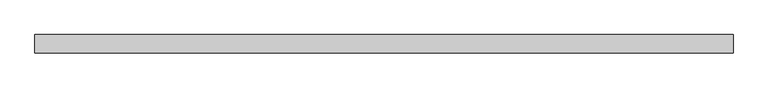
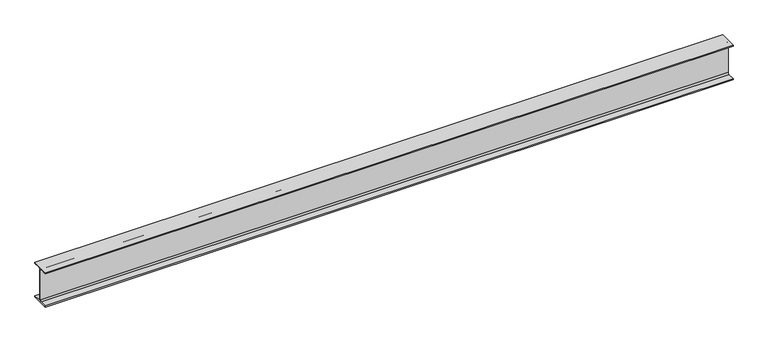
"""IFC4 building model written with IfcOpenShell, lengths in millimetres: beam geometry, 0912_Steel Framing_H-KSD3502 : H_SB_ASB_H-350x175x7x11."""

from ifc_helpers import new_model, si_unit, point, frame, frame_2d, origin, place, context, project, spatial, polyline, circle_curve, trimmed, segment, composite_curve, outline, extrude, source, transform, mapped, element, save


def beam_abbcd3b4(model_context):
    return source(origin(), model_context, "Body", "SweptSolid", [
        extrude(outline(composite_curve([segment(polyline([(87.5, -164.0), (87.5, -175.0), (-87.5, -175.0), (-87.5, -164.0), (-17.5, -164.0)]), True, "CONTINUOUS"), segment(trimmed(circle_curve(frame_2d((-17.5, -150.0)), 14.0), [point((-17.5, -164.0))], [point((-3.5, -150.0))], True, "CARTESIAN"), True, "CONTINUOUS"), segment(polyline([(-3.5, -150.0), (-3.5, 150.0)]), True, "CONTINUOUS"), segment(trimmed(circle_curve(frame_2d((-17.5, 150.0)), 14.0), [point((-3.5, 150.0))], [point((-17.5, 164.0))], True, "CARTESIAN"), True, "CONTINUOUS"), segment(polyline([(-17.5, 164.0), (-87.5, 164.0), (-87.5, 175.0), (87.5, 175.0), (87.5, 164.0), (17.5, 164.0)]), True, "CONTINUOUS"), segment(trimmed(circle_curve(frame_2d((17.5, 150.0)), 14.0), [point((17.5, 164.0))], [point((3.5, 150.0))], True, "CARTESIAN"), True, "CONTINUOUS"), segment(polyline([(3.5, 150.0), (3.5, -150.0)]), True, "CONTINUOUS"), segment(trimmed(circle_curve(frame_2d((17.5, -150.0)), 14.0), [point((3.5, -150.0))], [point((17.5, -164.0))], True, "CARTESIAN"), True, "CONTINUOUS"), segment(polyline([(17.5, -164.0), (87.5, -164.0)]), True, "CONTINUOUS")], self_intersect=False)), frame((-3262.3, 0.0, 0.0), z_axis=(1.0, 0.0, 0.0), x_axis=(0.0, 1.0, 0.0)), (0.0, 0.0, 1.0), 6599.6),
    ])


if __name__ == "__main__":
    model = new_model("IFC4")
    model_context = context("Model", 3, world=origin())
    ifc_project = project(units=[si_unit("LENGTHUNIT", "METRE", prefix="MILLI")], contexts=[model_context])
    site = spatial("IfcSite", under=ifc_project)
    building = spatial("IfcBuilding", under=site)
    placement = place(None, origin())
    beam_shape = beam_abbcd3b4(model_context)
    element("IfcBeam", 1, ObjectType="0912_Steel Framing_H-KSD3502 : H_SB_ASB_H-350x175x7x11", at=placement, inside=building, context=model_context, shape_type="MappedRepresentation", body=[
        mapped(beam_shape, transform((0.0, 0.0, 0.0), x_axis=(1.0, 0.0, 0.0), y_axis=(0.0, 1.0, 0.0), z_axis=(0.0, 0.0, 1.0))),
    ])
    save(model, "model.ifc")

# Revit data of these elements
# Type "0912_Steel Framing_H-KSD3502 : H_SB_ASB_H-350x175x7x11"
#   H_WM Code_1 = "S01AA002-00001 | Main Steel Structure Fabrication Work | Shelter/Building | Medium Steel - Standard (90KG/M>Weight≥30KG/M) | Material: (   )"
#   H_WM Code_2 = "S03AA028-00001 | Main Steel Structure Erection Work | Shelter/Building | Medium Steel (90KG/M>Weight≥30KG/M) | Material: (   )"
#   H_WM Code_3 = "S01AA010-00001 | Main Steel Structure Fabrication Work | Shelter/Building | Steel Painting/Coating | for Non-Fireproofed Steel Surface, Surface Preparation, Primer, Second & Final Coat | Material: (   )"
#   H_Q'ty Cal Type Tag = "SB-Q2"
#   Width = 17.5 cm
#   Web Thickness = 0.7 cm
#   Web Fillet = 1.4 cm
#   Warping Constant = 282000.0 cm⁶
#   W = 0
#   Torsional Moment of Inertia = 19.4042 cm⁴
#   Section Area = 63.14 cm²
#   Plastic Modulus weak axis = 174.0 cm³
#   Plastic Modulus strong axis = 868.0 cm³
#   Perimeter = 1.36 m²/m
#   Nominal Weight = 49.60 kgf/m
#   Moment of Inertia weak axis = 984.00 cm⁴
#   Moment of Inertia strong axis = 13600.00 cm⁴
#   Height = 35.0 cm
#   Flange Thickness = 1.1 cm
#   Elastic Modulus weak axis = 112.0 cm³
#   Elastic Modulus strong axis = 775.0 cm³
#   Centroid Vertical = 17.5 cm
#   Centroid Horizontal = 8.75 cm
#   Ix = 136000000
#   Length [instance default] = 1.5240 m
#   Zx = 868000
#   b = 0.1750 m
#   h = 0.3500 m
#   r = 0.0140 m
#   s = 0.0070 m
#   t = 0.0110 m
#   A = 0.006314 m²
#   Structural Material [instance default] = Steel, 45-345
#   Assembly Code = ""
# Element 1 (IfcBeam, "0912_Steel Framing_H-KSD3502 : H_SB_ASB_H-350x175x7x11")
#   Structural Material = none
# Materials
#   "Steel, 45-345": class "Metal", colour RGB 189 187 185, transparency 0, Description = "Steel 345 MPa", Cost = 0
